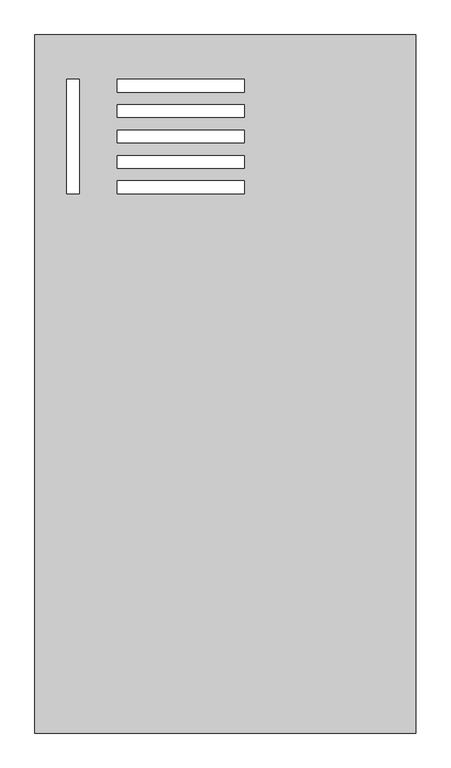
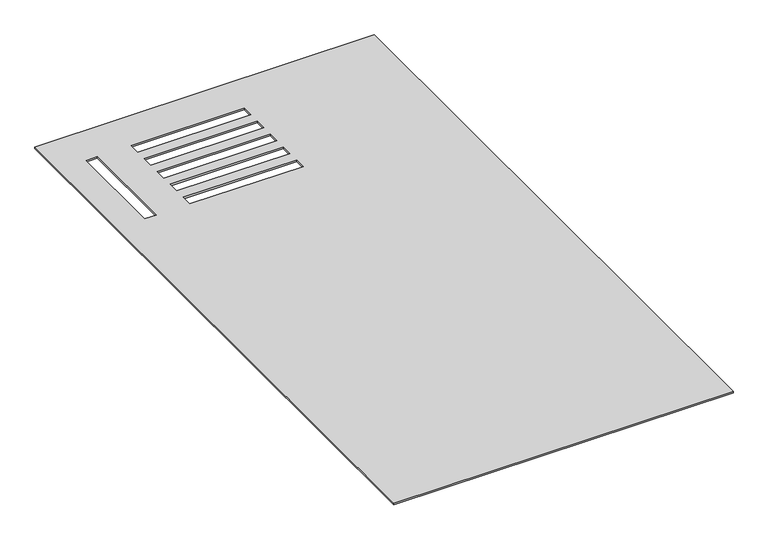
"""IFC4 building model written with IfcOpenShell, lengths in millimetres: proxy geometry, TSP Geyser Electrcical 150L : TSP Geyser Electrcical 150L."""

from ifc_helpers import new_model, si_unit, origin, origin_with_axes, place, context, project, spatial, polyline, outline, extrude, source, transform, mapped, element, save


def electrical_fixtures_357304c4(model_context):
    return source(origin(), model_context, "Body", "SweptSolid", [
        extrude(outline(polyline([(-600.0, 600.0), (0.0, 600.0), (0.0, -500.0), (-600.0, -500.0), (-600.0, 600.0)]), holes=[polyline([(-530.0, 530.0), (-550.0, 530.0), (-550.0, 350.0), (-530.0, 350.0), (-530.0, 530.0)]), polyline([(-470.0, 350.0), (-270.0, 350.0), (-270.0, 370.0), (-470.0, 370.0), (-470.0, 350.0)]), polyline([(-470.0, 390.0), (-270.0, 390.0), (-270.0, 410.0), (-470.0, 410.0), (-470.0, 390.0)]), polyline([(-470.0, 430.0), (-270.0, 430.0), (-270.0, 450.0), (-470.0, 450.0), (-470.0, 430.0)]), polyline([(-470.0, 470.0), (-270.0, 470.0), (-270.0, 490.0), (-470.0, 490.0), (-470.0, 470.0)]), polyline([(-470.0, 510.0), (-270.0, 510.0), (-270.0, 530.0), (-470.0, 530.0), (-470.0, 510.0)])]), origin_with_axes(), (0.0, 0.0, 1.0), 3.0),
    ])


if __name__ == "__main__":
    model = new_model("IFC4")
    model_context = context("Model", 3, world=origin())
    ifc_project = project(units=[si_unit("LENGTHUNIT", "METRE", prefix="MILLI")], contexts=[model_context])
    site = spatial("IfcSite", under=ifc_project)
    building = spatial("IfcBuilding", under=site)
    placement = place(None, origin())
    electrical_fixtures_shape = electrical_fixtures_357304c4(model_context)
    element("IfcBuildingElementProxy", 1, Name="TSP Geyser Electrcical 150L : TSP Geyser Electrcical 150L", ObjectType="TSP Geyser Electrcical 150L : TSP Geyser Electrcical 150L", at=placement, inside=building, context=model_context, shape_type="MappedRepresentation", body=[
        mapped(electrical_fixtures_shape, transform((0.0, 0.0, 0.0), x_axis=(1.0, 0.0, 0.0), y_axis=(0.0, 1.0, 0.0), z_axis=(0.0, 0.0, 1.0))),
    ])
    save(model, "model.ifc")

# Revit data of these elements
# Type "TSP Geyser Electrcical 150L : TSP Geyser Electrcical 150L"
#   Model = "TSP_EGEY150"
#   Default Elevation = 0
# Element 1 (IfcBuildingElementProxy, "TSP Geyser Electrcical 150L : TSP Geyser Electrcical 150L")
#   Materials on its faces: "Aluminum, Anodized Red"
# Materials
#   "Aluminum, Anodized Red": class "Metal", colour RGB 120 120 120, transparency 0, Description = "Anodized aluminum, red", Cost = 0
